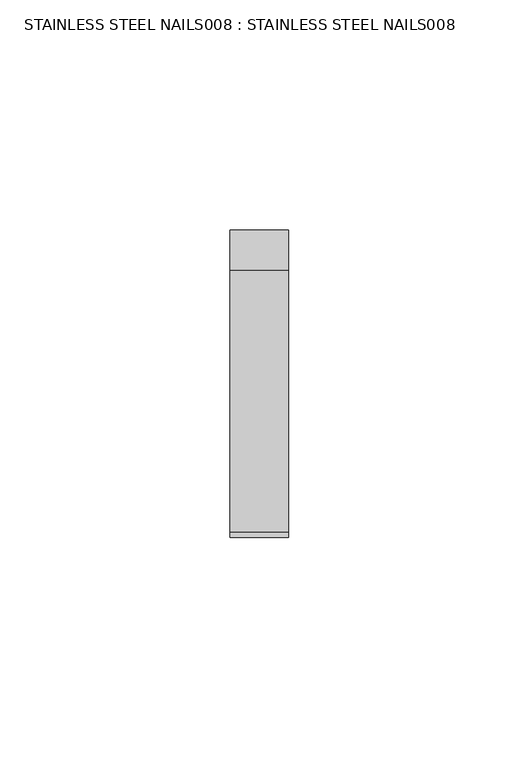
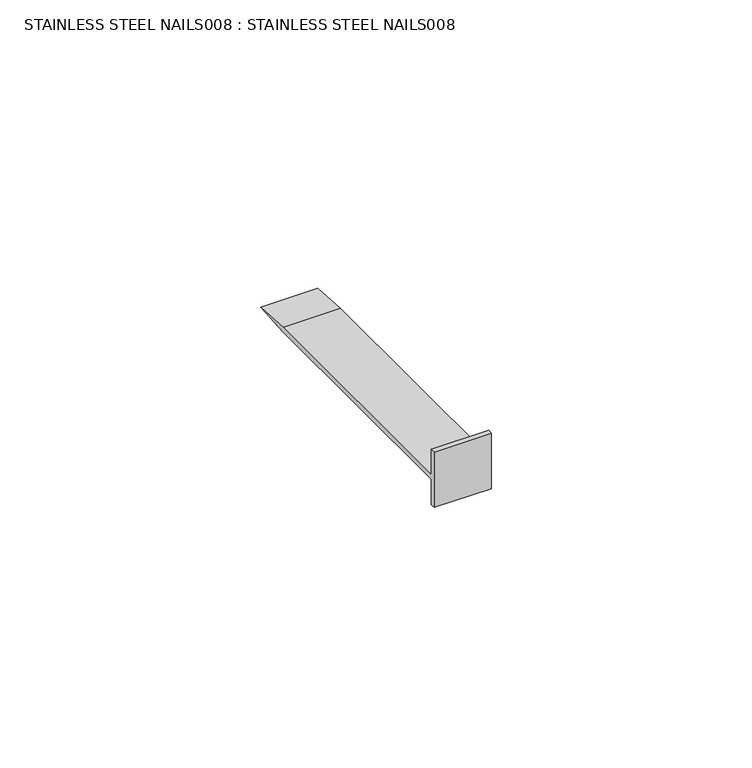
"""IFC4 building model written with IfcOpenShell, lengths in millimetres: proxy geometry, STAINLESS STEEL NAILS008 : STAINLESS STEEL NAILS008."""

import ifcopenshell
import ifcopenshell.guid

model = None  # the IFC model being written
_history = None  # IfcOwnerHistory: only IFC2X3 demands one
_inside = {}  # id of a spatial element -> (the spatial element, [elements in it])
_under = {}  # id of a project, library or spatial element -> (it, [spatial elements below it])
_declared = {}  # id of a project -> (the project, [libraries it declares])
_typed = {}  # id of a type object -> (the type object, [elements of that type])
_made_of = {}  # id of a material, layer set ... -> (it, [elements and type objects made of it])


def new_model(schema):
    """Start an empty IFC model of exactly this schema.

    Asked for "IFC4X3", IfcOpenShell would pick the latest addendum, in which some entities
    have other attributes; the version numbers below select the first issue.
    IFC2X3 requires an IfcOwnerHistory on every rooted entity: one is made here for all.
    """
    global model, _history
    if schema == "IFC4X3":
        model = ifcopenshell.file(schema_version=(4, 3, 0, 0))
    else:
        model = ifcopenshell.file(schema=schema)
    _inside.clear()
    _under.clear()
    _declared.clear()
    _typed.clear()
    _made_of.clear()
    _history = None
    if model.schema == "IFC2X3":
        org = make("IfcOrganization", Name="unknown")
        user = make(
            "IfcPersonAndOrganization",
            ThePerson=make("IfcPerson", FamilyName="unknown"),
            TheOrganization=org,
        )
        app = make(
            "IfcApplication",
            ApplicationDeveloper=org,
            Version="unknown",
            ApplicationFullName="unknown",
            ApplicationIdentifier="unknown",
        )
        _history = make(
            "IfcOwnerHistory",
            OwningUser=user,
            OwningApplication=app,
            ChangeAction="ADDED",
            CreationDate=0,
        )
    return model


def make(cls, **values):
    """One entity of the class cls with the attributes given. An attribute that is None is left unset."""
    return model.create_entity(
        cls, **{name: value for name, value in values.items() if value is not None}
    )


def rooted(cls, **values):
    """An entity with a GlobalId (a new one), such as an element, a storey or a relation."""
    return make(cls, GlobalId=ifcopenshell.guid.new(), OwnerHistory=_history, **values)


def si_unit(unit_type, name, prefix=None):
    """IfcSIUnit, for example si_unit("LENGTHUNIT", "METRE", prefix="MILLI")."""
    return make("IfcSIUnit", UnitType=unit_type, Prefix=prefix, Name=name)


def assignment(units):
    """IfcUnitAssignment: the units of a project."""
    return None if units is None else make("IfcUnitAssignment", Units=units)


def point(xyz):
    """IfcCartesianPoint."""
    return None if xyz is None else make("IfcCartesianPoint", Coordinates=xyz)


def direction(xyz):
    """IfcDirection."""
    return None if xyz is None else make("IfcDirection", DirectionRatios=xyz)


def frame(location, z_axis=None, x_axis=None):
    """IfcAxis2Placement3D, a coordinate frame: its origin and axes. An axis left out is left unset."""
    return make(
        "IfcAxis2Placement3D",
        Location=point(location),
        Axis=direction(z_axis),
        RefDirection=direction(x_axis),
    )


def origin():
    """The frame at (0, 0, 0) with its axes left unset."""
    return frame((0.0, 0.0, 0.0))


def place(relative_to, where):
    """IfcLocalPlacement: puts the frame where relative to a parent placement (None: the world)."""
    return make(
        "IfcLocalPlacement", PlacementRelTo=relative_to, RelativePlacement=where
    )


def context(
    kind, dimensions, precision=None, world=None, true_north=None, identifier=None
):
    """IfcGeometricRepresentationContext, for example the 3D "Model" context."""
    return make(
        "IfcGeometricRepresentationContext",
        ContextIdentifier=identifier,
        ContextType=kind,
        CoordinateSpaceDimension=dimensions,
        Precision=precision,
        WorldCoordinateSystem=world,
        TrueNorth=true_north,
    )


def project(units=None, contexts=None):
    """IfcProject with its units and contexts."""
    return rooted(
        "IfcProject",
        Name="project",
        RepresentationContexts=contexts,
        UnitsInContext=assignment(units),
    )


def spatial(cls, under=None, at=None, **own):
    """A site, building, storey or space (cls), placed at a placement, below another one or the project."""
    s = rooted(cls, ObjectPlacement=at, **own)
    if under is not None:
        _under.setdefault(under.id(), (under, []))[1].append(s)
    return s


def polyline(points):
    """IfcPolyline through the points."""
    return make("IfcPolyline", Points=[point(p) for p in points])


def outline(outer, holes=None, kind="AREA"):
    """IfcArbitraryClosedProfileDef: a profile drawn as a closed curve; with holes, ...WithVoids."""
    if holes is None:
        return make("IfcArbitraryClosedProfileDef", ProfileType=kind, OuterCurve=outer)
    return make(
        "IfcArbitraryProfileDefWithVoids",
        ProfileType=kind,
        OuterCurve=outer,
        InnerCurves=holes,
    )


def extrude(swept, where, along, depth):
    """IfcExtrudedAreaSolid: the profile swept, set in the frame where, extruded along a direction by depth."""
    return make(
        "IfcExtrudedAreaSolid",
        SweptArea=swept,
        Position=where,
        ExtrudedDirection=direction(along),
        Depth=depth,
    )


def shape(context_of_items, identifier, shape_type, items):
    """IfcShapeRepresentation: the items that make up one representation, for example the "Body"."""
    return make(
        "IfcShapeRepresentation",
        ContextOfItems=context_of_items,
        RepresentationIdentifier=identifier,
        RepresentationType=shape_type,
        Items=items,
    )


def source(mapping_origin, context_of_items, identifier, shape_type, items):
    """IfcRepresentationMap: a shape defined once, which mapped items show again and again."""
    return make(
        "IfcRepresentationMap",
        MappingOrigin=mapping_origin,
        MappedRepresentation=shape(context_of_items, identifier, shape_type, items),
    )


def transform(
    local_origin,
    x_axis=None,
    y_axis=None,
    z_axis=None,
    scale=None,
    scale2=None,
    scale3=None,
    uniform=True,
):
    """IfcCartesianTransformationOperator3D, or its non-uniform kind. x_axis, y_axis, z_axis: its Axis1, 2, 3."""
    if uniform:
        return make(
            "IfcCartesianTransformationOperator3D",
            Axis1=direction(x_axis),
            Axis2=direction(y_axis),
            LocalOrigin=point(local_origin),
            Scale=scale,
            Axis3=direction(z_axis),
        )
    return make(
        "IfcCartesianTransformationOperator3DnonUniform",
        Axis1=direction(x_axis),
        Axis2=direction(y_axis),
        LocalOrigin=point(local_origin),
        Scale=scale,
        Axis3=direction(z_axis),
        Scale2=scale2,
        Scale3=scale3,
    )


def mapped(mapping_source, mapping_target):
    """IfcMappedItem: shows the shape of a source again, moved by a transform."""
    return make(
        "IfcMappedItem", MappingSource=mapping_source, MappingTarget=mapping_target
    )


def made_of(thing, what):
    """Note that an element or type object is made of a material, layer set ...; save() writes the relation."""
    if what is not None:
        _made_of.setdefault(what.id(), (what, []))[1].append(thing)
    return thing


def element(
    cls,
    number,
    at=None,
    inside=None,
    cuts=None,
    type_object=None,
    material=None,
    context=None,
    identifier="Body",
    shape_type=None,
    held_by="IfcProductDefinitionShape",
    body=None,
    shapes=None,
    **own,
):
    """One element of the class cls, such as IfcWall. Its Tag is "e" and its number.

    at: its placement. inside: the storey or other place that contains it. cuts: it is an
    opening in that element (IfcRelVoidsElement). A single representation is given by context,
    identifier, shape_type and body (its items); several are given by shapes. held_by: the class
    of the entity that holds the representations. save() writes the other relations.
    """
    e = rooted(cls, Tag="e%d" % number, ObjectPlacement=at, **own)
    if body is not None:
        shapes = [shape(context, identifier, shape_type, body)]
    if shapes is not None:
        e.Representation = make(held_by, Representations=shapes)
    if inside is not None:
        _inside.setdefault(inside.id(), (inside, []))[1].append(e)
    if cuts is not None:
        rooted(
            "IfcRelVoidsElement", RelatingBuildingElement=cuts, RelatedOpeningElement=e
        )
    if type_object is not None:
        _typed.setdefault(type_object.id(), (type_object, []))[1].append(e)
    return made_of(e, material)


def aggregate(whole, parts):
    """IfcRelAggregates: a whole, such as a stair, and the parts it consists of."""
    return rooted("IfcRelAggregates", RelatingObject=whole, RelatedObjects=parts)


def save(model, path):
    """Write the relations noted so far, then the file.

    IfcRelAggregates (storeys below a building ...), IfcRelContainedInSpatialStructure (elements
    in a storey), IfcRelDefinesByType, IfcRelAssociatesMaterial and IfcRelDeclares: one each for
    every whole, place, type object, material and project.
    """
    for whole, parts in _under.values():
        aggregate(whole, parts)
    for where, things in _inside.values():
        rooted(
            "IfcRelContainedInSpatialStructure",
            RelatedElements=things,
            RelatingStructure=where,
        )
    for kind, things in _typed.values():
        rooted("IfcRelDefinesByType", RelatedObjects=things, RelatingType=kind)
    for what, things in _made_of.values():
        rooted("IfcRelAssociatesMaterial", RelatedObjects=things, RelatingMaterial=what)
    for by, libraries in _declared.values():
        rooted("IfcRelDeclares", RelatingContext=by, RelatedDefinitions=libraries)
    model.write(path)


def stainless_steel_nails008_stainless_steel_nails008_ed18b8cf(model_context):
    return source(origin(), model_context, "Body", "SweptSolid", [
        extrude(outline(polyline([(-5577.378205, 40134.3588724), (-5577.378205, 40147.3572563), (-5576.2950063, 40147.3572563), (-5576.2950063, 40141.3996637), (-5519.393468, 40141.3996637), (-5510.7278788, 40140.8591651), (-5519.4110792, 40140.316465), (-5576.2950063, 40140.316465), (-5576.2950063, 40134.3588724), (-5577.378205, 40134.3588724)])), frame((14383.0178845, 0.0, 0.0), z_axis=(1.0, 0.0, 0.0), x_axis=(0.0, 1.0, 0.0)), (0.0, 0.0, 1.0), 12.7),
    ])


if __name__ == "__main__":
    model = new_model("IFC4")
    model_context = context("Model", 3, world=origin())
    ifc_project = project(units=[si_unit("LENGTHUNIT", "METRE", prefix="MILLI")], contexts=[model_context])
    site = spatial("IfcSite", under=ifc_project)
    building = spatial("IfcBuilding", under=site)
    placement = place(None, origin())
    stainless_steel_nails008_stainless_steel_nails008_shape = stainless_steel_nails008_stainless_steel_nails008_ed18b8cf(model_context)
    element("IfcBuildingElementProxy", 1, Name="STAINLESS STEEL NAILS008 : STAINLESS STEEL NAILS008", ObjectType="STAINLESS STEEL NAILS008 : STAINLESS STEEL NAILS008", at=placement, inside=building, context=model_context, shape_type="MappedRepresentation", body=[
        mapped(stainless_steel_nails008_stainless_steel_nails008_shape, transform((0.0, 0.0, 0.0), x_axis=(1.0, 0.0, 0.0), y_axis=(0.0, 1.0, 0.0), z_axis=(0.0, 0.0, 1.0))),
    ])
    save(model, "model.ifc")

# Revit data of these elements
# Type "STAINLESS STEEL NAILS008 : STAINLESS STEEL NAILS008"
#   NameOverride = "STAINLESS STEEL NAILS008"
# Element 1 (IfcBuildingElementProxy, "STAINLESS STEEL NAILS008 : STAINLESS STEEL NAILS008")
#   Materials on its faces: "1 3/4\" STAINLESS STEEL RINGSHANK 5D COMMON NAILS @ 4\" (101.6MM) O.C. FIRESTONE PROVIDED MAX., 1/2\" STAGGERED"
# Materials
#   "1 3/4\" STAINLESS STEEL RINGSHANK 5D COMMON NAILS @ 4\" (101.6MM) O.C. FIRESTONE PROVIDED MAX., 1/2\" STAGGERED": class "Unassigned", colour RGB 255 255 255, transparency 0
